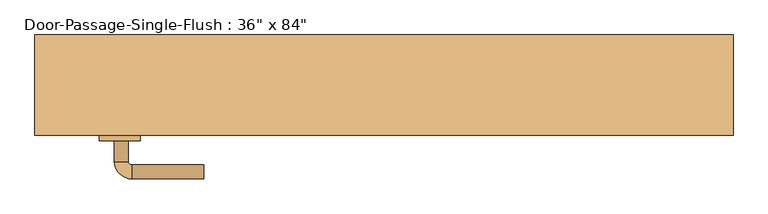
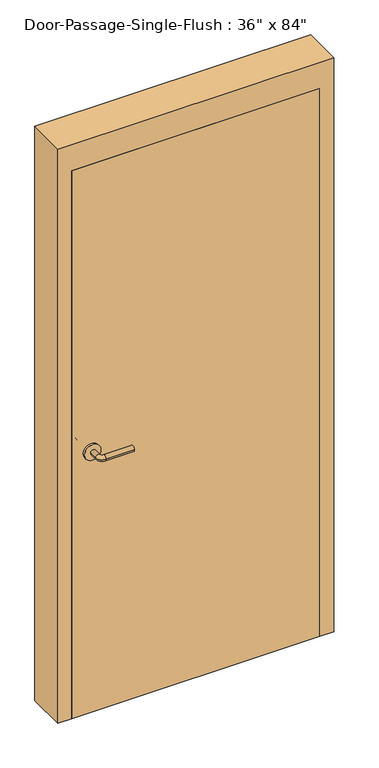
"""IFC4 building model written with IfcOpenShell, lengths in millimetres: door geometry."""

from ifc_helpers import new_model, si_unit, point, frame, frame_2d, origin, origin_with_axes, place, context, project, spatial, polyline, circle_curve, ellipse_curve, trimmed, segment, composite_curve, outline, extrude, faceted_brep, source, transform, mapped, element, save
from ifc_brep_helpers import plane_surface, cylinder_surface, revolved_surface, advanced_brep


def door_58febf71(model_context):
    return source(origin(), model_context, "Body", "SolidModel", [
        advanced_brep(
        [(-392.190625, -76.1375, 1016.0), (-372.190625, -76.1375, 1016.0), (-392.190625, -46.1375, 1016.0), (-372.190625, -46.1375, 1016.0), (-367.190625, -41.1375, 1016.0), (-367.190625, -21.1375, 1016.0), (-262.190625, -21.1375, 1016.0), (-262.190625, -41.1375, 1016.0)],
        [
            (0, 1, circle_curve(frame((-382.190625, -76.1375, 1016.0), z_axis=(0.0, -1.0, 0.0), x_axis=(1.0, 0.0, 0.0)), 10.0)),
            (1, 0, circle_curve(frame((-382.190625, -76.1375, 1016.0), z_axis=(0.0, -1.0, 0.0), x_axis=(1.0, 0.0, 0.0)), 10.0)),
            (0, 2),
            (2, 3, circle_curve(frame((-382.190625, -46.1375, 1016.0), z_axis=(0.0, -1.0, 0.0), x_axis=(1.0, 0.0, 0.0)), 10.0)),
            (3, 1),
            (3, 2, circle_curve(frame((-382.190625, -46.1375, 1016.0), z_axis=(0.0, -1.0, 0.0), x_axis=(1.0, 0.0, 0.0)), 10.0)),
            (4, 3, circle_curve(frame((-367.190625, -46.1375, 1016.0), z_axis=(0.0, 0.0, 1.0), x_axis=(-1.0, 0.0, 0.0)), 5.0)),
            (2, 5, circle_curve(frame((-367.190625, -46.1375, 1016.0), z_axis=(0.0, 0.0, -1.0), x_axis=(-1.0, 0.0, 0.0)), 25.0)),
            (5, 4, circle_curve(frame((-367.190625, -31.1375, 1016.0), z_axis=(-1.0, 0.0, 0.0), x_axis=(0.0, -1.0, 0.0)), 10.0)),
            (4, 5, circle_curve(frame((-367.190625, -31.1375, 1016.0), z_axis=(-1.0, 0.0, 0.0), x_axis=(0.0, -1.0, 0.0)), 10.0)),
            (6, 7, circle_curve(frame((-262.190625, -31.1375, 1016.0), z_axis=(1.0, 0.0, 0.0), x_axis=(0.0, -1.0, 0.0)), 10.0)),
            (7, 6, circle_curve(frame((-262.190625, -31.1375, 1016.0), z_axis=(1.0, 0.0, 0.0), x_axis=(0.0, -1.0, 0.0)), 10.0)),
            (5, 6),
            (7, 4),
        ],
        [
            plane_surface(frame((-382.190625, -76.1375, 1016.0), z_axis=(0.0, -1.0, 0.0), x_axis=(0.0, 0.0, 1.0))),
            cylinder_surface(frame((-382.190625, -76.1375, 1016.0), z_axis=(0.0, -1.0, 0.0), x_axis=(1.0, 0.0, 0.0)), 10.0),
            revolved_surface(trimmed(ellipse_curve(frame((-382.190625, -46.1375, 1016.0), z_axis=(0.0, -1.0, 0.0), x_axis=(1.0, 0.0, 0.0)), 10.0, 10.0), [point((-392.190625, -46.1375, 1016.0))], [point((-372.190625, -46.1375, 1016.0))], True, "CARTESIAN"), (-367.190625, -46.1375, 1016.0), (0.0, 0.0, -1.0)),
            revolved_surface(trimmed(ellipse_curve(frame((-382.190625, -46.1375, 1016.0), z_axis=(0.0, -1.0, 0.0), x_axis=(1.0, 0.0, 0.0)), 10.0, 10.0), [point((-372.190625, -46.1375, 1016.0))], [point((-392.190625, -46.1375, 1016.0))], True, "CARTESIAN"), (-367.190625, -46.1375, 1016.0), (0.0, 0.0, -1.0)),
            plane_surface(frame((-262.190625, -31.1375, 1016.0), z_axis=(1.0, 0.0, 0.0), x_axis=(0.0, 0.0, 1.0))),
            cylinder_surface(frame((-367.190625, -31.1375, 1016.0), z_axis=(-1.0, 0.0, 0.0), x_axis=(0.0, -1.0, 0.0)), 10.0),
        ],
        [
            (0, [[1, 2]]),
            (1, [[-1, 3, 4, 5]]),
            (1, [[-2, -5, 6, -3]]),
            (2, [[7, -4, 8, 9]]),
            (3, [[-8, -6, -7, 10]]),
            (4, [[11, 12]]),
            (5, [[-9, 13, -12, 14]]),
            (5, [[-10, -14, -11, -13]]),
        ],
    ),
        extrude(outline(composite_curve([segment(trimmed(circle_curve(frame_2d((1016.0, -384.690625)), 30.0), [point((1016.0, -414.690625))], [point((1016.0, -354.690625))], False, "CARTESIAN"), True, "CONTINUOUS"), segment(trimmed(circle_curve(frame_2d((1016.0, -384.690625)), 30.0), [point((1016.0, -354.690625))], [point((1016.0, -414.690625))], False, "CARTESIAN"), True, "CONTINUOUS")], self_intersect=False)), frame((0.0, -84.1375, 0.0), z_axis=(0.0, 1.0, 0.0), x_axis=(0.0, 0.0, 1.0)), (0.0, 0.0, 1.0), 8.0),
        advanced_brep(
        [(-392.190625, -136.5875, 1016.0), (-372.190625, -136.5875, 1016.0), (-372.190625, -166.5875, 1016.0), (-392.190625, -166.5875, 1016.0), (-367.190625, -171.5875, 1016.0), (-367.190625, -191.5875, 1016.0), (-262.190625, -191.5875, 1016.0), (-262.190625, -171.5875, 1016.0)],
        [
            (0, 1, circle_curve(frame((-382.190625, -136.5875, 1016.0), z_axis=(0.0, 1.0, 0.0), x_axis=(1.0, 0.0, 0.0)), 10.0)),
            (1, 0, circle_curve(frame((-382.190625, -136.5875, 1016.0), z_axis=(0.0, 1.0, 0.0), x_axis=(1.0, 0.0, 0.0)), 10.0)),
            (1, 2),
            (2, 3, circle_curve(frame((-382.190625, -166.5875, 1016.0), z_axis=(0.0, 1.0, 0.0), x_axis=(1.0, 0.0, 0.0)), 10.0)),
            (3, 0),
            (3, 2, circle_curve(frame((-382.190625, -166.5875, 1016.0), z_axis=(0.0, 1.0, 0.0), x_axis=(1.0, 0.0, 0.0)), 10.0)),
            (4, 5, circle_curve(frame((-367.190625, -181.5875, 1016.0), z_axis=(-1.0, 0.0, 0.0), x_axis=(0.0, 1.0, 0.0)), 10.0)),
            (5, 3, circle_curve(frame((-367.190625, -166.5875, 1016.0), z_axis=(0.0, 0.0, -1.0), x_axis=(-1.0, 0.0, 0.0)), 25.0)),
            (2, 4, circle_curve(frame((-367.190625, -166.5875, 1016.0), z_axis=(0.0, 0.0, 1.0), x_axis=(-1.0, 0.0, 0.0)), 5.0)),
            (5, 4, circle_curve(frame((-367.190625, -181.5875, 1016.0), z_axis=(-1.0, 0.0, 0.0), x_axis=(0.0, 1.0, 0.0)), 10.0)),
            (6, 7, circle_curve(frame((-262.190625, -181.5875, 1016.0), z_axis=(1.0, 0.0, 0.0), x_axis=(0.0, 1.0, 0.0)), 10.0)),
            (7, 6, circle_curve(frame((-262.190625, -181.5875, 1016.0), z_axis=(1.0, 0.0, 0.0), x_axis=(0.0, 1.0, 0.0)), 10.0)),
            (4, 7),
            (6, 5),
        ],
        [
            plane_surface(frame((-382.190625, -136.5875, 1016.0), z_axis=(0.0, 1.0, 0.0), x_axis=(0.0, 0.0, 1.0))),
            cylinder_surface(frame((-382.190625, -136.5875, 1016.0), z_axis=(0.0, 1.0, 0.0), x_axis=(1.0, 0.0, 0.0)), 10.0),
            revolved_surface(trimmed(ellipse_curve(frame((-382.190625, -166.5875, 1016.0), z_axis=(0.0, -1.0, 0.0), x_axis=(1.0, 0.0, 0.0)), 10.0, 10.0), [point((-392.190625, -166.5875, 1016.0))], [point((-372.190625, -166.5875, 1016.0))], True, "CARTESIAN"), (-367.190625, -166.5875, 1016.0), (0.0, 0.0, -1.0)),
            revolved_surface(trimmed(ellipse_curve(frame((-382.190625, -166.5875, 1016.0), z_axis=(0.0, -1.0, 0.0), x_axis=(1.0, 0.0, 0.0)), 10.0, 10.0), [point((-372.190625, -166.5875, 1016.0))], [point((-392.190625, -166.5875, 1016.0))], True, "CARTESIAN"), (-367.190625, -166.5875, 1016.0), (0.0, 0.0, -1.0)),
            plane_surface(frame((-262.190625, -181.5875, 1016.0), z_axis=(1.0, 0.0, 0.0), x_axis=(0.0, 0.0, 1.0))),
            cylinder_surface(frame((-367.190625, -181.5875, 1016.0), z_axis=(-1.0, 0.0, 0.0), x_axis=(0.0, 1.0, 0.0)), 10.0),
        ],
        [
            (0, [[1, 2]]),
            (1, [[3, 4, 5, -2]]),
            (1, [[-5, 6, -3, -1]]),
            (2, [[7, 8, -4, 9]]),
            (3, [[10, -9, -6, -8]]),
            (4, [[11, 12]]),
            (5, [[13, -11, 14, -7]]),
            (5, [[-14, -12, -13, -10]]),
        ],
    ),
        extrude(outline(composite_curve([segment(trimmed(circle_curve(frame_2d((1016.0, -384.690625)), 30.0), [point((1016.0, -414.690625))], [point((1016.0, -354.690625))], False, "CARTESIAN"), True, "CONTINUOUS"), segment(trimmed(circle_curve(frame_2d((1016.0, -384.690625)), 30.0), [point((1016.0, -354.690625))], [point((1016.0, -414.690625))], False, "CARTESIAN"), True, "CONTINUOUS")], self_intersect=False)), frame((0.0, -136.5875, 0.0), z_axis=(0.0, 1.0, 0.0), x_axis=(0.0, 0.0, 1.0)), (0.0, 0.0, 1.0), 8.0),
        faceted_brep([(457.2, -79.375, 0.0), (441.325, -79.375, 0.0), (441.325, -31.75, 0.0), (457.2, -31.75, 0.0), (457.2, 17.4625, 0.0), (508.0, 17.4625, 0.0), (508.0, -128.5875, 0.0), (457.2, -128.5875, 0.0), (457.2, -128.5875, 2133.6), (457.2, -79.375, 2133.6), (508.0, -128.5875, 2235.2), (-508.0, -128.5875, 2235.2), (-508.0, -128.5875, 0.0), (-457.2, -128.5875, 0.0), (-457.2, -128.5875, 2133.6), (508.0, 17.4625, 2235.2), (457.2, 17.4625, 2133.6), (-457.2, 17.4625, 2133.6), (-457.2, 17.4625, 0.0), (-508.0, 17.4625, 0.0), (-508.0, 17.4625, 2235.2), (457.2, -31.75, 2133.6), (441.325, -31.75, 2117.725), (-441.325, -31.75, 2117.725), (-441.325, -31.75, 0.0), (-457.2, -31.75, 0.0), (-457.2, -31.75, 2133.6), (441.325, -79.375, 2117.725), (-457.2, -79.375, 2133.6), (-457.2, -79.375, 0.0), (-441.325, -79.375, 0.0), (-441.325, -79.375, 2117.725)], [[[0, 1, 2, 3, 4, 5, 6, 7]], [[7, 8, 9, 0]], [[6, 10, 11, 12, 13, 14, 8, 7]], [[5, 15, 10, 6]], [[4, 16, 17, 18, 19, 20, 15, 5]], [[3, 21, 16, 4]], [[2, 22, 23, 24, 25, 26, 21, 3]], [[1, 27, 22, 2]], [[0, 9, 28, 29, 30, 31, 27, 1]], [[8, 14, 28, 9]], [[16, 21, 26, 17]], [[22, 27, 31, 23]], [[12, 19, 18, 25, 24, 30, 29, 13]], [[13, 29, 28, 14]], [[11, 20, 19, 12]], [[17, 26, 25, 18]], [[23, 31, 30, 24]], [[15, 20, 11, 10]]]),
        extrude(outline(polyline([(457.2, -84.1375), (457.2, -128.5875), (-457.2, -128.5875), (-457.2, -84.1375), (457.2, -84.1375)])), origin_with_axes(), (0.0, 0.0, 1.0), 2133.6),
    ])


if __name__ == "__main__":
    model = new_model("IFC4")
    model_context = context("Model", 3, world=origin())
    ifc_project = project(units=[si_unit("LENGTHUNIT", "METRE", prefix="MILLI")], contexts=[model_context])
    site = spatial("IfcSite", under=ifc_project)
    building = spatial("IfcBuilding", under=site)
    placement = place(None, origin())
    door_shape = door_58febf71(model_context)
    element("IfcDoor", 1, ObjectType="Door-Passage-Single-Flush : 36\" x 84\"", at=placement, inside=building, context=model_context, shape_type="MappedRepresentation", body=[
        mapped(door_shape, transform((0.0, 0.0, 0.0), x_axis=(1.0, 0.0, 0.0), y_axis=(0.0, 1.0, 0.0), z_axis=(0.0, 0.0, 1.0))),
    ])
    save(model, "model.ifc")

# Revit data of these elements
# Type "Door-Passage-Single-Flush : 36\" x 84\""
#   Type Mark = "1"
#   Assembly Code = "B2030200"
#   Analytic Construction = "Wooden"
#   Thickness = 0' - 1 3/4"
#   Thermal Resistance (R) = 2.5876 (h·ft²·°F)/BTU
#   Swing Angle [instance default] = 90.00°
#   Strike Height = 3' - 4"
#   Rough Width [instance default] = 3' - 4"
#   Rough Height [instance default] = 7' - 4"
#   MF Opening Height [instance default] = 0' - 4"
#   MF Opening Width [instance default] = 0' - 4"
#   Inset Calculate [instance default] = 0' - 4"
#   Masonry Inset [instance default] = 0' - 1"
#   Height = 7' - 0"
#   Width = 3' - 0"
#   Heat Transfer Coefficient (U) = 0.3865 BTU/(h·ft²·°F)
#   Masonry Frame Depth = 0' - 5 3/4"
#   Define Thermal Properties by = 1
#   Masonry Frame [instance default] = yes
#   Function = 1
#   Dry Wall Frame [instance default] = no
#   Panel Material = Wood - Birch
#   Frame Material = Metal - Paint Finish - Grey
#   Door Handle Material = Aluminum
#   Visual Light Transmittance = 0
#   Solar Heat Gain Coefficient = 0
#   Wall Closure = (empty or 0)
# Element 1 (IfcDoor, "Door-Passage-Single-Flush : 36\" x 84\"")
#   Materials on its faces: "Aluminum", "Metal - Paint Finish - Grey", "Wood - Birch"
# Materials
#   "Wood - Birch": class "Wood", colour RGB 166 116 52, transparency 0, Cost = 0
#   "Metal - Paint Finish - Grey": class "Paint", colour RGB 104 104 104, transparency 0, Cost = 0
#   "Aluminum": class "Metal", colour RGB 247 247 247, transparency 0, Description = "Aluminum 6061", Cost = 0
